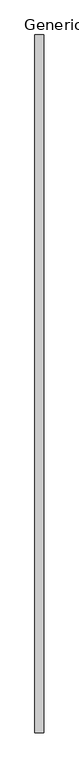
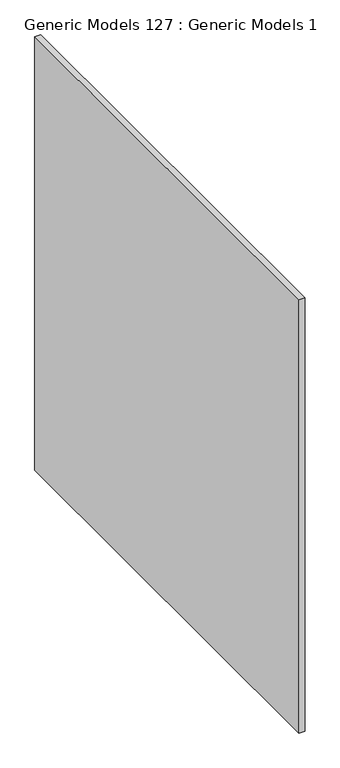
"""IFC4 building model written with IfcOpenShell, lengths in millimetres: proxy geometry, Generic Models 127 : Generic Models 1."""

from ifc_helpers import new_model, si_unit, frame, origin, place, context, project, spatial, polyline, outline, extrude, source, transform, mapped, element, save


def generic_models_127_generic_models_1_8e526843(model_context):
    return source(origin(), model_context, "Body", "SweptSolid", [
        extrude(outline(polyline([(46827.9235531, 1219.2), (46843.7985531, 1219.2), (46843.7985531, 0.0), (46827.9235531, 0.0), (46827.9235531, 1219.2)])), frame((0.0, 0.0, 999.573933), z_axis=(0.0, 0.0, 1.0), x_axis=(1.0, 0.0, 0.0)), (0.0, 0.0, 1.0), 1219.2),
    ])


if __name__ == "__main__":
    model = new_model("IFC4")
    model_context = context("Model", 3, world=origin())
    ifc_project = project(units=[si_unit("LENGTHUNIT", "METRE", prefix="MILLI")], contexts=[model_context])
    site = spatial("IfcSite", under=ifc_project)
    building = spatial("IfcBuilding", under=site)
    placement = place(None, origin())
    generic_models_127_generic_models_1_shape = generic_models_127_generic_models_1_8e526843(model_context)
    element("IfcBuildingElementProxy", 1, Name="Generic Models 127 : Generic Models 1", ObjectType="Generic Models 127 : Generic Models 1", at=placement, inside=building, context=model_context, shape_type="MappedRepresentation", body=[
        mapped(generic_models_127_generic_models_1_shape, transform((0.0, 0.0, 0.0), x_axis=(1.0, 0.0, 0.0), y_axis=(0.0, 1.0, 0.0), z_axis=(0.0, 0.0, 1.0))),
    ])
    save(model, "model.ifc")

# Revit data of these elements
# Element 1 (IfcBuildingElementProxy, "Generic Models 127 : Generic Models 1")
#   Materials on its faces: "5/8\" GYP. BD"
# Materials
#   "5/8\" GYP. BD": class "Generic", colour RGB 255 255 255, transparency 0, Description = "Gypsum Wall Board", Cost = 0
